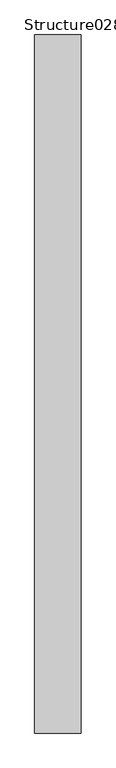
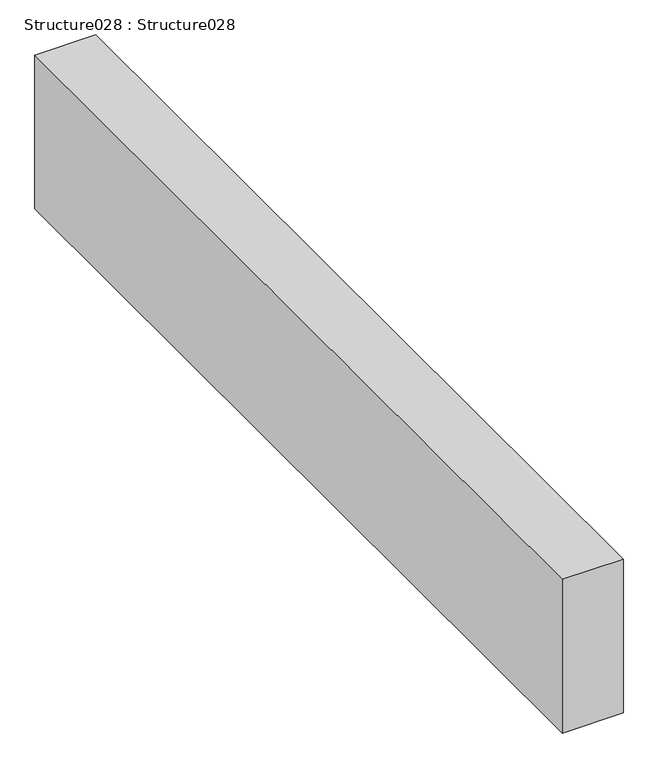
"""IFC4 building model written with IfcOpenShell, lengths in millimetres: proxy geometry, Structure028 : Structure028."""

from ifc_helpers import new_model, si_unit, frame, origin, place, context, project, spatial, polyline, outline, extrude, source, transform, mapped, element, save


def structure028_structure028_2ddeed53(model_context):
    return source(origin(), model_context, "Body", "SweptSolid", [
        extrude(outline(polyline([(-9434.8987014, 7982.1531721), (-9568.2487014, 7982.1531721), (-9568.2487014, 9982.1531721), (-9434.8987014, 9982.1531721), (-9434.8987014, 7982.1531721)])), frame((0.0, 0.0, 39579.2960083), z_axis=(0.0, 0.0, 1.0), x_axis=(1.0, 0.0, 0.0)), (0.0, 0.0, 1.0), 355.6),
    ])


if __name__ == "__main__":
    model = new_model("IFC4")
    model_context = context("Model", 3, world=origin())
    ifc_project = project(units=[si_unit("LENGTHUNIT", "METRE", prefix="MILLI")], contexts=[model_context])
    site = spatial("IfcSite", under=ifc_project)
    building = spatial("IfcBuilding", under=site)
    placement = place(None, origin())
    structure028_structure028_shape = structure028_structure028_2ddeed53(model_context)
    element("IfcBuildingElementProxy", 1, Name="Structure028 : Structure028", ObjectType="Structure028 : Structure028", at=placement, inside=building, context=model_context, shape_type="MappedRepresentation", body=[
        mapped(structure028_structure028_shape, transform((0.0, 0.0, 0.0), x_axis=(1.0, 0.0, 0.0), y_axis=(0.0, 1.0, 0.0), z_axis=(0.0, 0.0, 1.0))),
    ])
    save(model, "model.ifc")

# Revit data of these elements
# Type "Structure028 : Structure028"
#   NameOverride = "Structure028"
# Element 1 (IfcBuildingElementProxy, "Structure028 : Structure028")
#   Materials on its faces: "STRUCTURAL MEMBER (SEE STRUCTURAL DWGS)"
# Materials
#   "STRUCTURAL MEMBER (SEE STRUCTURAL DWGS)": class "Unassigned", colour RGB 176 134 95, transparency 0, Cost = 0
